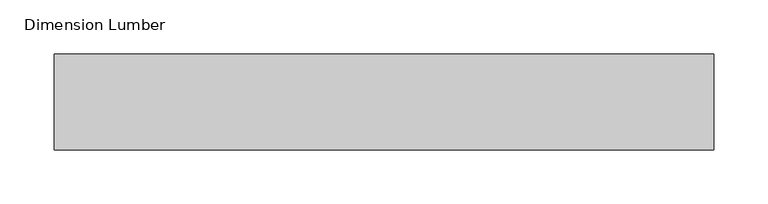
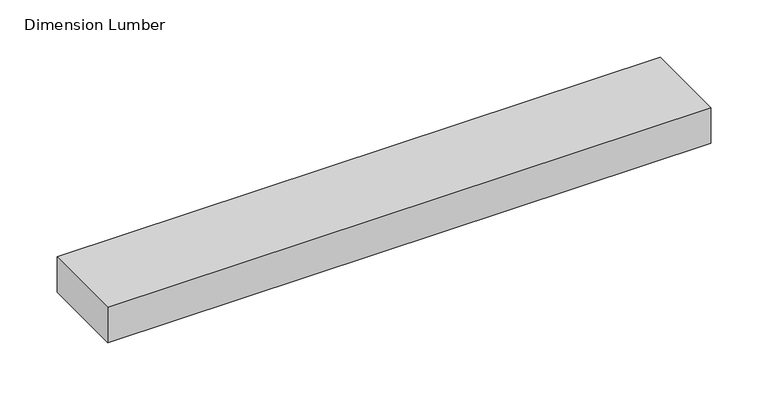
"""IFC4 building model written with IfcOpenShell, lengths in millimetres: beam geometry, Dimension Lumber : Opening Plate 2*4 Exterior."""

from ifc_helpers import new_model, si_unit, frame, origin, place, context, project, spatial, polyline, outline, extrude, source, transform, mapped, element, save


def dimension_lumber_0879c48f(model_context):
    return source(origin(), model_context, "Body", "SweptSolid", [
        extrude(outline(polyline([(304.8, 44.45), (304.8, -44.45), (-304.8, -44.45), (-304.8, 44.45), (304.8, 44.45)])), frame((0.0, 0.0, -19.05), z_axis=(0.0, 0.0, 1.0), x_axis=(1.0, 0.0, 0.0)), (0.0, 0.0, 1.0), 38.1),
    ])


if __name__ == "__main__":
    model = new_model("IFC4")
    model_context = context("Model", 3, world=origin())
    ifc_project = project(units=[si_unit("LENGTHUNIT", "METRE", prefix="MILLI")], contexts=[model_context])
    site = spatial("IfcSite", under=ifc_project)
    building = spatial("IfcBuilding", under=site)
    placement = place(None, origin())
    dimension_lumber_shape = dimension_lumber_0879c48f(model_context)
    element("IfcBeam", 1, ObjectType="Dimension Lumber : Opening Plate 2*4 Exterior", at=placement, inside=building, context=model_context, shape_type="MappedRepresentation", body=[
        mapped(dimension_lumber_shape, transform((0.0, 0.0, 0.0), x_axis=(1.0, 0.0, 0.0), y_axis=(0.0, 1.0, 0.0), z_axis=(0.0, 0.0, 1.0))),
    ])
    save(model, "model.ifc")

# Revit data of these elements
# Type "Dimension Lumber : Opening Plate 2*4 Exterior"
#   Assembly Code = "B10"
#   A = 0.0364583 SF
#   Length [instance default] = 5' - 0"
#   b = 0' - 3 1/2"
#   d = 0' - 1 1/2"
#   Structural Material [instance default] = Softwood, Lumber
# Element 1 (IfcBeam, "Dimension Lumber : Opening Plate 2*4 Exterior")
#   Structural Material = Douglas Fir #2
#   Materials on its faces: "Douglas Fir #2"
# Materials
#   "Softwood, Lumber": class "Wood", colour RGB 223 192 134, transparency 0, Description = "Pinus Echinata", Cost = 0
#   "Douglas Fir #2": class "Wood", colour RGB 223 192 134, transparency 0, Description = "Pinus Echinata", Cost = 0
